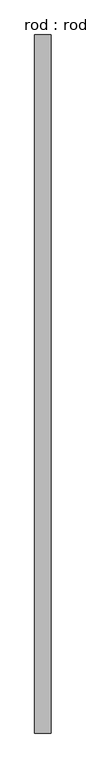
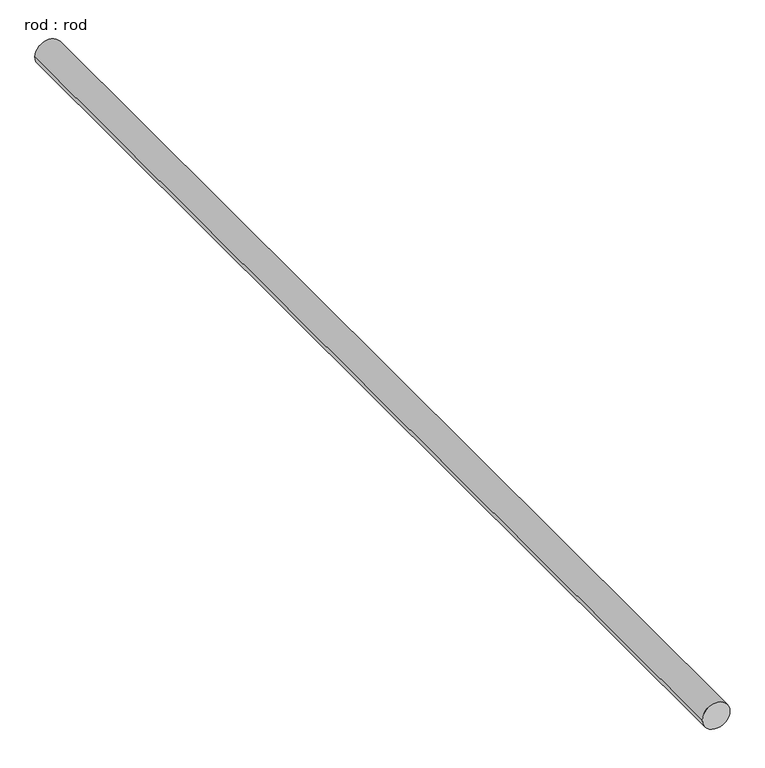
"""IFC4 building model written with IfcOpenShell, lengths in millimetres: proxy geometry, rod : rod."""

from ifc_helpers import new_model, si_unit, point, frame, frame_2d, origin, place, context, project, spatial, circle_curve, trimmed, segment, composite_curve, outline, extrude, source, transform, mapped, element, save


def rod_rod_79d0ea63(model_context):
    return source(origin(), model_context, "Body", "SweptSolid", [
        extrude(outline(composite_curve([segment(trimmed(circle_curve(frame_2d((0.0108462, 0.0)), 200.0), [point((0.0108462, 200.0))], [point((0.0108462, -200.0))], False, "CARTESIAN"), True, "CONTINUOUS"), segment(trimmed(circle_curve(frame_2d((0.0108462, 0.0)), 200.0), [point((0.0108462, -200.0))], [point((0.0108462, 200.0))], False, "CARTESIAN"), True, "CONTINUOUS")], self_intersect=False)), frame((0.0, -4323.8755221, 0.0), z_axis=(0.0, 1.0, 0.0), x_axis=(0.0, 0.0, 1.0)), (0.0, 0.0, 1.0), 16833.2082749),
    ])


if __name__ == "__main__":
    model = new_model("IFC4")
    model_context = context("Model", 3, world=origin())
    ifc_project = project(units=[si_unit("LENGTHUNIT", "METRE", prefix="MILLI")], contexts=[model_context])
    site = spatial("IfcSite", under=ifc_project)
    building = spatial("IfcBuilding", under=site)
    placement = place(None, origin())
    rod_rod_shape = rod_rod_79d0ea63(model_context)
    element("IfcBuildingElementProxy", 1, Name="rod : rod", ObjectType="rod : rod", at=placement, inside=building, context=model_context, shape_type="MappedRepresentation", body=[
        mapped(rod_rod_shape, transform((0.0, 0.0, 0.0), x_axis=(1.0, 0.0, 0.0), y_axis=(0.0, 1.0, 0.0), z_axis=(0.0, 0.0, 1.0))),
    ])
    save(model, "model.ifc")

# Revit data of these elements
# Type "rod : rod"
#   Default Elevation = 0
